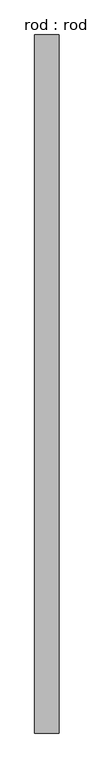
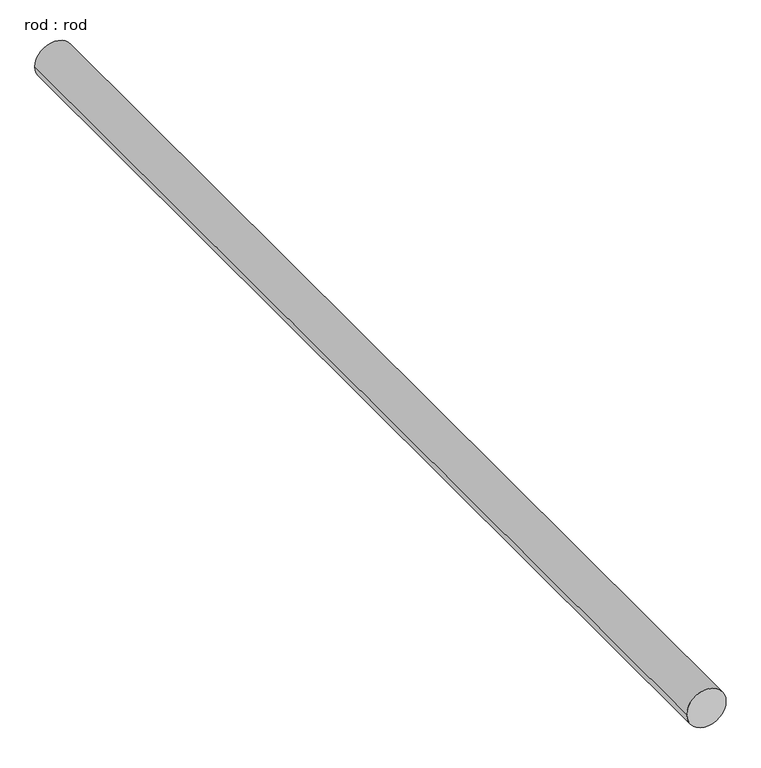
"""IFC4 building model written with IfcOpenShell, lengths in millimetres: proxy geometry, rod : rod."""

from ifc_helpers import new_model, si_unit, point, frame, frame_2d, origin, place, context, project, spatial, circle_curve, trimmed, segment, composite_curve, outline, extrude, source, transform, mapped, element, save


def rod_rod_81fdb6b2(model_context):
    return source(origin(), model_context, "Body", "SweptSolid", [
        extrude(outline(composite_curve([segment(trimmed(circle_curve(frame_2d((0.0108462, 0.0)), 200.0), [point((0.0108462, 200.0))], [point((0.0108462, -200.0))], False, "CARTESIAN"), True, "CONTINUOUS"), segment(trimmed(circle_curve(frame_2d((0.0108462, 0.0)), 200.0), [point((0.0108462, -200.0))], [point((0.0108462, 200.0))], False, "CARTESIAN"), True, "CONTINUOUS")], self_intersect=False)), frame((0.0, -1657.2713847, 0.0), z_axis=(0.0, 1.0, 0.0), x_axis=(0.0, 0.0, 1.0)), (0.0, 0.0, 1.0), 11500.0),
    ])


if __name__ == "__main__":
    model = new_model("IFC4")
    model_context = context("Model", 3, world=origin())
    ifc_project = project(units=[si_unit("LENGTHUNIT", "METRE", prefix="MILLI")], contexts=[model_context])
    site = spatial("IfcSite", under=ifc_project)
    building = spatial("IfcBuilding", under=site)
    placement = place(None, origin())
    rod_rod_shape = rod_rod_81fdb6b2(model_context)
    element("IfcBuildingElementProxy", 1, Name="rod : rod", ObjectType="rod : rod", at=placement, inside=building, context=model_context, shape_type="MappedRepresentation", body=[
        mapped(rod_rod_shape, transform((0.0, 0.0, 0.0), x_axis=(1.0, 0.0, 0.0), y_axis=(0.0, 1.0, 0.0), z_axis=(0.0, 0.0, 1.0))),
    ])
    save(model, "model.ifc")

# Revit data of these elements
# Type "rod : rod"
#   Default Elevation = 0
